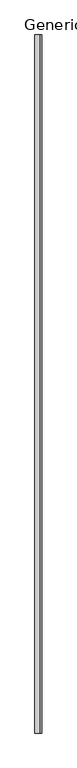
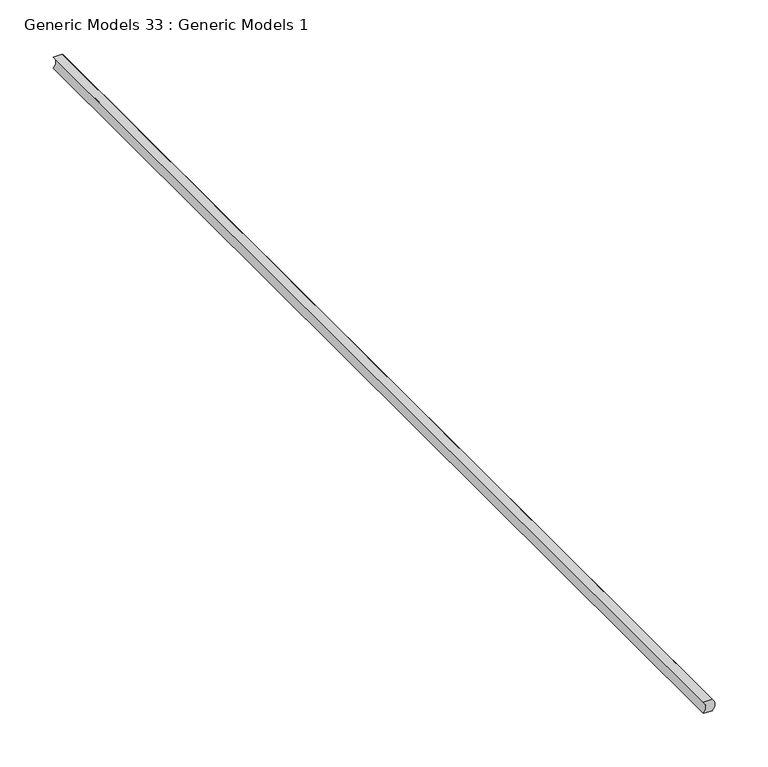
"""IFC4 building model written with IfcOpenShell, lengths in millimetres: proxy geometry, Generic Models 33 : Generic Models 1."""

from ifc_helpers import new_model, si_unit, point, frame, frame_2d, origin, place, context, project, spatial, polyline, circle_curve, trimmed, segment, composite_curve, outline, extrude, source, transform, mapped, element, save


def generic_models_33_generic_models_1_084f7e48(model_context):
    return source(origin(), model_context, "Body", "SweptSolid", [
        extrude(outline(composite_curve([segment(polyline([(2438.4, 48444.15), (2438.4, 48453.675)]), True, "CONTINUOUS"), segment(trimmed(circle_curve(frame_2d((2444.75, 48447.845519)), 8.620055), [point((2438.4, 48453.675))], [point((2451.1, 48453.675))], False, "CARTESIAN"), True, "CONTINUOUS"), segment(polyline([(2451.1, 48453.675), (2451.1, 48444.15)]), True, "CONTINUOUS"), segment(trimmed(circle_curve(frame_2d((2444.75, 48438.320519)), 8.620055), [point((2451.1, 48444.15))], [point((2438.4, 48444.15))], True, "CARTESIAN"), True, "CONTINUOUS")], self_intersect=False)), frame((0.0, 0.0, 0.0), z_axis=(0.0, 1.0, 0.0), x_axis=(0.0, 0.0, 1.0)), (0.0, 0.0, 1.0), 1219.2),
    ])


if __name__ == "__main__":
    model = new_model("IFC4")
    model_context = context("Model", 3, world=origin())
    ifc_project = project(units=[si_unit("LENGTHUNIT", "METRE", prefix="MILLI")], contexts=[model_context])
    site = spatial("IfcSite", under=ifc_project)
    building = spatial("IfcBuilding", under=site)
    placement = place(None, origin())
    generic_models_33_generic_models_1_shape = generic_models_33_generic_models_1_084f7e48(model_context)
    element("IfcBuildingElementProxy", 1, Name="Generic Models 33 : Generic Models 1", ObjectType="Generic Models 33 : Generic Models 1", at=placement, inside=building, context=model_context, shape_type="MappedRepresentation", body=[
        mapped(generic_models_33_generic_models_1_shape, transform((0.0, 0.0, 0.0), x_axis=(1.0, 0.0, 0.0), y_axis=(0.0, 1.0, 0.0), z_axis=(0.0, 0.0, 1.0))),
    ])
    save(model, "model.ifc")

# Revit data of these elements
# Element 1 (IfcBuildingElementProxy, "Generic Models 33 : Generic Models 1")
#   Materials on its faces: "ACOUSTICAL SEALANT"
# Materials
#   "ACOUSTICAL SEALANT": class "Unassigned", colour RGB 120 120 120, transparency 0, Cost = 0
